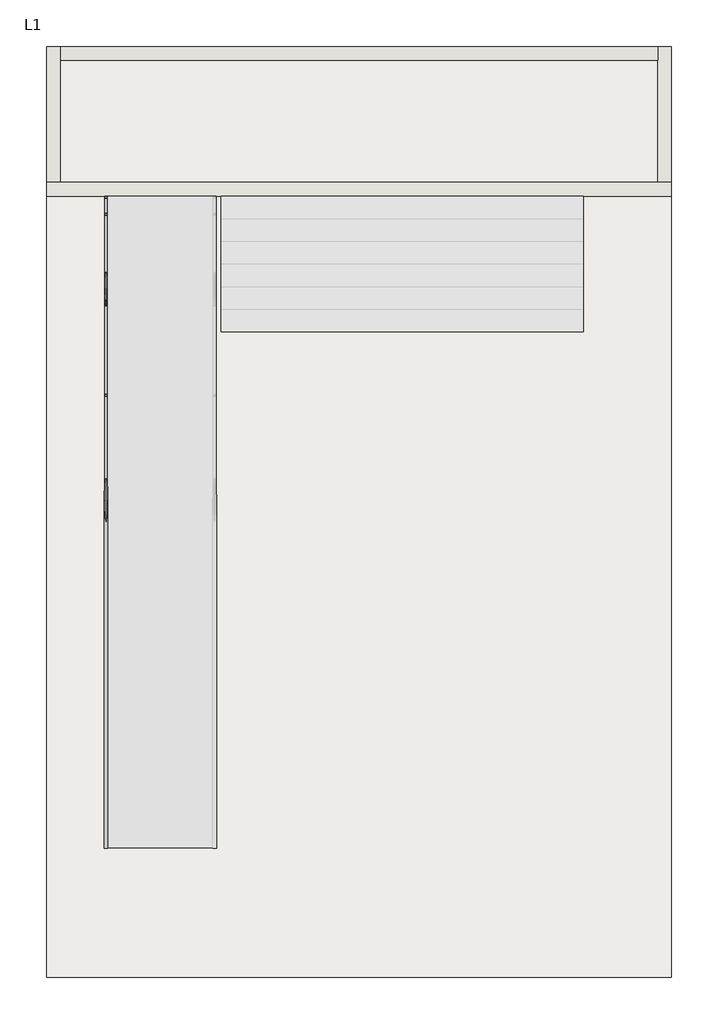
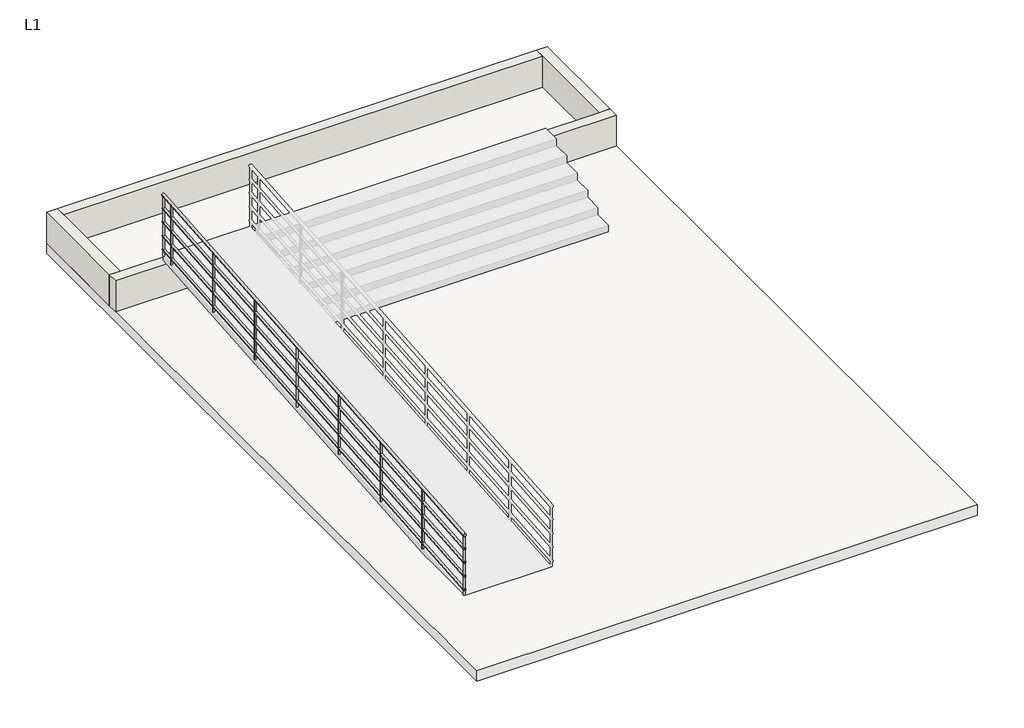
# One storey, part 1 of 2: 4 walls, 1 railing, 1 slab.
"""IFC4 building model written with IfcOpenShell, lengths in millimetres."""

from ifc_helpers import new_model, si_unit, frame, origin, origin_with_axes, place, context, project, spatial, polyline, ellipse_curve, outline, extrude, faceted_brep, element, save
from ifc_brep_helpers import plane_surface, cylinder_surface, advanced_brep

model = new_model("IFC4")

# Units and contexts
model_context = context("Model", 3, world=origin())
ifc_project = project(units=[si_unit("LENGTHUNIT", "METRE", prefix="MILLI")], contexts=[model_context])

# Site, building, storey
site = spatial("IfcSite", under=ifc_project)
building = spatial("IfcBuilding", under=site)
storey = spatial("IfcBuildingStorey", under=building, Name="L1", Elevation=0.0)

# Railing
placement = place(None, origin())
element("IfcRailing", 1, ObjectType="900mm Pipe", at=placement, inside=storey, context=model_context, shape_type="AdvancedBrep", body=[
    advanced_brep(
    [(-579.8488078, -8058.4292912, 879.9306757), (-619.8488078, -8058.4292912, 879.9306757), (-579.8488078, -858.4292912, 1479.9306757), (-619.8488078, -858.4292912, 1479.9306757)],
    [
        (0, 1, ellipse_curve(frame((-599.8488078, -8058.4292912, 879.9306757), z_axis=(0.0, -1.0, 0.0), x_axis=(0.0, 0.0, -1.0)), 20.0693243, 20.0)),
        (1, 0, ellipse_curve(frame((-599.8488078, -8058.4292912, 879.9306757), z_axis=(0.0, -1.0, 0.0), x_axis=(0.0, 0.0, -1.0)), 20.0693243, 20.0)),
        (2, 3, ellipse_curve(frame((-599.8488078, -858.4292912, 1479.9306757), z_axis=(0.0, 1.0, 0.0), x_axis=(0.0, 0.0, -1.0)), 20.0693243, 20.0)),
        (3, 2, ellipse_curve(frame((-599.8488078, -858.4292912, 1479.9306757), z_axis=(0.0, 1.0, 0.0), x_axis=(0.0, 0.0, -1.0)), 20.0693243, 20.0)),
        (0, 2),
        (3, 1),
    ],
    [
        plane_surface(frame((-599.8488078, -8058.4292912, 900.0), z_axis=(0.0, -1.0, 0.0), x_axis=(0.0, 0.0, 1.0))),
        plane_surface(frame((-599.8488078, -858.4292912, 1500.0), z_axis=(0.0, 1.0, 0.0), x_axis=(0.0, 0.0, 1.0))),
        cylinder_surface(frame((-599.8488078, -8056.7683816, 880.0690848), z_axis=(0.0, -0.9965457582448797, -0.08304547985373999), x_axis=(-1.0, 0.0, 0.0)), 20.0),
    ],
    [
        (0, [[1, 2]]),
        (1, [[3, 4]]),
        (2, [[-1, 5, -4, 6]]),
        (2, [[-2, -6, -3, -5]]),
    ],
),
    advanced_brep(
    [(-614.8488078, -8058.4292912, 684.9480068), (-584.8488078, -8058.4292912, 684.9480068), (-614.8488078, -858.4292912, 1284.9480068), (-584.8488078, -858.4292912, 1284.9480068)],
    [
        (0, 1, ellipse_curve(frame((-599.8488078, -8058.4292912, 684.9480068), z_axis=(0.0, -1.0, 0.0), x_axis=(0.0, 0.0, -0.9999999999999999)), 15.0519932, 15.0)),
        (1, 0, ellipse_curve(frame((-599.8488078, -8058.4292912, 684.9480068), z_axis=(0.0, -1.0, 0.0), x_axis=(0.0, 0.0, -0.9999999999999999)), 15.0519932, 15.0)),
        (2, 3, ellipse_curve(frame((-599.8488078, -858.4292912, 1284.9480068), z_axis=(0.0, 1.0, 0.0), x_axis=(0.0, 0.0, -0.9999999999999999)), 15.0519932, 15.0)),
        (3, 2, ellipse_curve(frame((-599.8488078, -858.4292912, 1284.9480068), z_axis=(0.0, 1.0, 0.0), x_axis=(0.0, 0.0, -0.9999999999999999)), 15.0519932, 15.0)),
        (0, 2),
        (3, 1),
    ],
    [
        plane_surface(frame((-599.8488078, -8058.4292912, 700.0), z_axis=(0.0, -1.0, 0.0), x_axis=(0.0, 0.0, 1.0))),
        plane_surface(frame((-599.8488078, -858.4292912, 1300.0), z_axis=(0.0, 1.0, 0.0), x_axis=(0.0, 0.0, 1.0))),
        cylinder_surface(frame((-599.8488078, -8057.183609, 685.0518136), z_axis=(0.0, -0.9965457582448797, -0.08304547985373997), x_axis=(1.0, 0.0, 0.0)), 15.0),
    ],
    [
        (0, [[1, 2]]),
        (1, [[3, 4]]),
        (2, [[-1, 5, -4, 6]]),
        (2, [[-2, -6, -3, -5]]),
    ],
),
    advanced_brep(
    [(-614.8488078, -8058.4292912, 484.9480068), (-584.8488078, -8058.4292912, 484.9480068), (-614.8488078, -858.4292912, 1084.9480068), (-584.8488078, -858.4292912, 1084.9480068)],
    [
        (0, 1, ellipse_curve(frame((-599.8488078, -8058.4292912, 484.9480068), z_axis=(0.0, -1.0, 0.0), x_axis=(0.0, 0.0, -0.9999999999999999)), 15.0519932, 15.0)),
        (1, 0, ellipse_curve(frame((-599.8488078, -8058.4292912, 484.9480068), z_axis=(0.0, -1.0, 0.0), x_axis=(0.0, 0.0, -0.9999999999999999)), 15.0519932, 15.0)),
        (2, 3, ellipse_curve(frame((-599.8488078, -858.4292912, 1084.9480068), z_axis=(0.0, 1.0, 0.0), x_axis=(0.0, 0.0, -0.9999999999999999)), 15.0519932, 15.0)),
        (3, 2, ellipse_curve(frame((-599.8488078, -858.4292912, 1084.9480068), z_axis=(0.0, 1.0, 0.0), x_axis=(0.0, 0.0, -0.9999999999999999)), 15.0519932, 15.0)),
        (0, 2),
        (3, 1),
    ],
    [
        plane_surface(frame((-599.8488078, -8058.4292912, 500.0), z_axis=(0.0, -1.0, 0.0), x_axis=(0.0, 0.0, 1.0))),
        plane_surface(frame((-599.8488078, -858.4292912, 1100.0), z_axis=(0.0, 1.0, 0.0), x_axis=(0.0, 0.0, 1.0))),
        cylinder_surface(frame((-599.8488078, -8057.183609, 485.0518136), z_axis=(0.0, -0.9965457582448797, -0.08304547985373997), x_axis=(1.0, 0.0, 0.0)), 15.0),
    ],
    [
        (0, [[1, 2]]),
        (1, [[3, 4]]),
        (2, [[-1, 5, -4, 6]]),
        (2, [[-2, -6, -3, -5]]),
    ],
),
    advanced_brep(
    [(-614.8488078, -8058.4292912, 284.9480068), (-584.8488078, -8058.4292912, 284.9480068), (-614.8488078, -858.4292912, 884.9480068), (-584.8488078, -858.4292912, 884.9480068)],
    [
        (0, 1, ellipse_curve(frame((-599.8488078, -8058.4292912, 284.9480068), z_axis=(0.0, -1.0, 0.0), x_axis=(0.0, 0.0, -0.9999999999999999)), 15.0519932, 15.0)),
        (1, 0, ellipse_curve(frame((-599.8488078, -8058.4292912, 284.9480068), z_axis=(0.0, -1.0, 0.0), x_axis=(0.0, 0.0, -0.9999999999999999)), 15.0519932, 15.0)),
        (2, 3, ellipse_curve(frame((-599.8488078, -858.4292912, 884.9480068), z_axis=(0.0, 1.0, 0.0), x_axis=(0.0, 0.0, -0.9999999999999999)), 15.0519932, 15.0)),
        (3, 2, ellipse_curve(frame((-599.8488078, -858.4292912, 884.9480068), z_axis=(0.0, 1.0, 0.0), x_axis=(0.0, 0.0, -0.9999999999999999)), 15.0519932, 15.0)),
        (0, 2),
        (3, 1),
    ],
    [
        plane_surface(frame((-599.8488078, -8058.4292912, 300.0), z_axis=(0.0, -1.0, 0.0), x_axis=(0.0, 0.0, 1.0))),
        plane_surface(frame((-599.8488078, -858.4292912, 900.0), z_axis=(0.0, 1.0, 0.0), x_axis=(0.0, 0.0, 1.0))),
        cylinder_surface(frame((-599.8488078, -8057.183609, 285.0518136), z_axis=(0.0, -0.9965457582448797, -0.08304547985373997), x_axis=(1.0, 0.0, 0.0)), 15.0),
    ],
    [
        (0, [[1, 2]]),
        (1, [[3, 4]]),
        (2, [[-1, 5, -4, 6]]),
        (2, [[-2, -6, -3, -5]]),
    ],
),
    advanced_brep(
    [(-614.8488078, -8058.4292912, 84.9480068), (-584.8488078, -8058.4292912, 84.9480068), (-614.8488078, -858.4292912, 684.9480068), (-584.8488078, -858.4292912, 684.9480068)],
    [
        (0, 1, ellipse_curve(frame((-599.8488078, -8058.4292912, 84.9480068), z_axis=(0.0, -1.0, 0.0), x_axis=(0.0, 0.0, -0.9999999999999999)), 15.0519932, 15.0)),
        (1, 0, ellipse_curve(frame((-599.8488078, -8058.4292912, 84.9480068), z_axis=(0.0, -1.0, 0.0), x_axis=(0.0, 0.0, -0.9999999999999999)), 15.0519932, 15.0)),
        (2, 3, ellipse_curve(frame((-599.8488078, -858.4292912, 684.9480068), z_axis=(0.0, 1.0, 0.0), x_axis=(0.0, 0.0, -0.9999999999999999)), 15.0519932, 15.0)),
        (3, 2, ellipse_curve(frame((-599.8488078, -858.4292912, 684.9480068), z_axis=(0.0, 1.0, 0.0), x_axis=(0.0, 0.0, -0.9999999999999999)), 15.0519932, 15.0)),
        (0, 2),
        (3, 1),
    ],
    [
        plane_surface(frame((-599.8488078, -8058.4292912, 100.0), z_axis=(0.0, -1.0, 0.0), x_axis=(0.0, 0.0, 1.0))),
        plane_surface(frame((-599.8488078, -858.4292912, 700.0), z_axis=(0.0, 1.0, 0.0), x_axis=(0.0, 0.0, 1.0))),
        cylinder_surface(frame((-599.8488078, -8057.183609, 85.0518136), z_axis=(0.0, -0.9965457582448797, -0.08304547985373997), x_axis=(1.0, 0.0, 0.0)), 15.0),
    ],
    [
        (0, [[1, 2]]),
        (1, [[3, 4]]),
        (2, [[-1, 5, -4, 6]]),
        (2, [[-2, -6, -3, -5]]),
    ],
),
    advanced_brep(
    [(-587.3488078, -1058.4292912, 1443.1946847), (-587.3488078, -1058.4292912, 583.3333333), (-612.3488078, -1058.4292912, 583.3333333), (-612.3488078, -1058.4292912, 1443.1946847)],
    [
        (0, 1),
        (1, 2, ellipse_curve(frame((-599.8488078, -1058.4292912, 583.3333333), z_axis=(0.0, -0.08304547985373995, 0.9965457582448797), x_axis=(0.0, 0.9965457582448798, 0.08304547985373882)), 12.5433277, 12.5)),
        (2, 3),
        (3, 0, ellipse_curve(frame((-599.8488078, -1058.4292912, 1443.1946847), z_axis=(0.0, 0.08304547985373997, -0.9965457582448797), x_axis=(0.0, 0.9965457582448797, 0.0830454798537388)), 12.5433277, 12.5)),
        (0, 3, ellipse_curve(frame((-599.8488078, -1058.4292912, 1443.1946847), z_axis=(0.0, 0.08304547985373997, -0.9965457582448797), x_axis=(0.0, 0.9965457582448797, 0.0830454798537388)), 12.5433277, 12.5)),
        (2, 1, ellipse_curve(frame((-599.8488078, -1058.4292912, 583.3333333), z_axis=(0.0, -0.08304547985373995, 0.9965457582448797), x_axis=(0.0, 0.9965457582448798, 0.08304547985373882)), 12.5433277, 12.5)),
    ],
    [
        cylinder_surface(frame((-599.8488078, -1058.4292912, 483.3333333), z_axis=(0.0, 0.0, 1.0), x_axis=(-1.0, 0.0, 0.0)), 12.5),
        plane_surface(frame((-624.8488078, -1033.4292912, 1445.2780181), z_axis=(0.0, -0.08304547985373997, 0.9965457582448797), x_axis=(1.0, 0.0, 0.0))),
        plane_surface(frame((-624.8488078, -1083.4292912, 581.25), z_axis=(0.0, 0.08304547985373995, -0.9965457582448797), x_axis=(1.0, 0.0, 0.0))),
    ],
    [
        (0, [[1, 2, 3, 4]]),
        (0, [[-1, 5, -3, 6]]),
        (1, [[-4, -5]]),
        (2, [[-2, -6]]),
    ],
),
    advanced_brep(
    [(-587.3488078, -2058.4292912, 1359.8613514), (-587.3488078, -2058.4292912, 500.0), (-612.3488078, -2058.4292912, 500.0), (-612.3488078, -2058.4292912, 1359.8613514)],
    [
        (0, 1),
        (1, 2, ellipse_curve(frame((-599.8488078, -2058.4292912, 500.0), z_axis=(0.0, -0.08304547985373995, 0.9965457582448797), x_axis=(0.0, 0.9965457582448798, 0.08304547985373882)), 12.5433277, 12.5)),
        (2, 3),
        (3, 0, ellipse_curve(frame((-599.8488078, -2058.4292912, 1359.8613514), z_axis=(0.0, 0.08304547985373997, -0.9965457582448797), x_axis=(0.0, 0.9965457582448797, 0.0830454798537388)), 12.5433277, 12.5)),
        (0, 3, ellipse_curve(frame((-599.8488078, -2058.4292912, 1359.8613514), z_axis=(0.0, 0.08304547985373997, -0.9965457582448797), x_axis=(0.0, 0.9965457582448797, 0.0830454798537388)), 12.5433277, 12.5)),
        (2, 1, ellipse_curve(frame((-599.8488078, -2058.4292912, 500.0), z_axis=(0.0, -0.08304547985373995, 0.9965457582448797), x_axis=(0.0, 0.9965457582448798, 0.08304547985373882)), 12.5433277, 12.5)),
    ],
    [
        cylinder_surface(frame((-599.8488078, -2058.4292912, 400.0), z_axis=(0.0, 0.0, 1.0), x_axis=(-1.0, 0.0, 0.0)), 12.5),
        plane_surface(frame((-624.8488078, -2033.4292912, 1361.9446847), z_axis=(0.0, -0.08304547985373997, 0.9965457582448797), x_axis=(1.0, 0.0, 0.0))),
        plane_surface(frame((-624.8488078, -2083.4292912, 497.9166667), z_axis=(0.0, 0.08304547985373995, -0.9965457582448797), x_axis=(1.0, 0.0, 0.0))),
    ],
    [
        (0, [[1, 2, 3, 4]]),
        (0, [[-1, 5, -3, 6]]),
        (1, [[-4, -5]]),
        (2, [[-2, -6]]),
    ],
),
    advanced_brep(
    [(-587.3488078, -3058.4292912, 1276.5280181), (-587.3488078, -3058.4292912, 416.6666667), (-612.3488078, -3058.4292912, 416.6666667), (-612.3488078, -3058.4292912, 1276.5280181)],
    [
        (0, 1),
        (1, 2, ellipse_curve(frame((-599.8488078, -3058.4292912, 416.6666667), z_axis=(0.0, -0.08304547985373995, 0.9965457582448797), x_axis=(0.0, 0.9965457582448798, 0.08304547985373882)), 12.5433277, 12.5)),
        (2, 3),
        (3, 0, ellipse_curve(frame((-599.8488078, -3058.4292912, 1276.5280181), z_axis=(0.0, 0.08304547985373997, -0.9965457582448797), x_axis=(0.0, 0.9965457582448797, 0.0830454798537388)), 12.5433277, 12.5)),
        (0, 3, ellipse_curve(frame((-599.8488078, -3058.4292912, 1276.5280181), z_axis=(0.0, 0.08304547985373997, -0.9965457582448797), x_axis=(0.0, 0.9965457582448797, 0.0830454798537388)), 12.5433277, 12.5)),
        (2, 1, ellipse_curve(frame((-599.8488078, -3058.4292912, 416.6666667), z_axis=(0.0, -0.08304547985373995, 0.9965457582448797), x_axis=(0.0, 0.9965457582448798, 0.08304547985373882)), 12.5433277, 12.5)),
    ],
    [
        cylinder_surface(frame((-599.8488078, -3058.4292912, 316.6666667), z_axis=(0.0, 0.0, 1.0), x_axis=(-1.0, 0.0, 0.0)), 12.5),
        plane_surface(frame((-624.8488078, -3033.4292912, 1278.6113514), z_axis=(0.0, -0.08304547985373997, 0.9965457582448797), x_axis=(1.0, 0.0, 0.0))),
        plane_surface(frame((-624.8488078, -3083.4292912, 414.5833333), z_axis=(0.0, 0.08304547985373995, -0.9965457582448797), x_axis=(1.0, 0.0, 0.0))),
    ],
    [
        (0, [[1, 2, 3, 4]]),
        (0, [[-1, 5, -3, 6]]),
        (1, [[-4, -5]]),
        (2, [[-2, -6]]),
    ],
),
    advanced_brep(
    [(-587.3488078, -4058.4292912, 1193.1946847), (-587.3488078, -4058.4292912, 333.3333333), (-612.3488078, -4058.4292912, 333.3333333), (-612.3488078, -4058.4292912, 1193.1946847)],
    [
        (0, 1),
        (1, 2, ellipse_curve(frame((-599.8488078, -4058.4292912, 333.3333333), z_axis=(0.0, -0.08304547985373995, 0.9965457582448797), x_axis=(0.0, 0.9965457582448798, 0.08304547985373882)), 12.5433277, 12.5)),
        (2, 3),
        (3, 0, ellipse_curve(frame((-599.8488078, -4058.4292912, 1193.1946847), z_axis=(0.0, 0.08304547985373997, -0.9965457582448797), x_axis=(0.0, 0.9965457582448797, 0.0830454798537388)), 12.5433277, 12.5)),
        (0, 3, ellipse_curve(frame((-599.8488078, -4058.4292912, 1193.1946847), z_axis=(0.0, 0.08304547985373997, -0.9965457582448797), x_axis=(0.0, 0.9965457582448797, 0.0830454798537388)), 12.5433277, 12.5)),
        (2, 1, ellipse_curve(frame((-599.8488078, -4058.4292912, 333.3333333), z_axis=(0.0, -0.08304547985373995, 0.9965457582448797), x_axis=(0.0, 0.9965457582448798, 0.08304547985373882)), 12.5433277, 12.5)),
    ],
    [
        cylinder_surface(frame((-599.8488078, -4058.4292912, 233.3333333), z_axis=(0.0, 0.0, 1.0), x_axis=(-1.0, 0.0, 0.0)), 12.5),
        plane_surface(frame((-624.8488078, -4033.4292912, 1195.2780181), z_axis=(0.0, -0.08304547985373997, 0.9965457582448797), x_axis=(1.0, 0.0, 0.0))),
        plane_surface(frame((-624.8488078, -4083.4292912, 331.25), z_axis=(0.0, 0.08304547985373995, -0.9965457582448797), x_axis=(1.0, 0.0, 0.0))),
    ],
    [
        (0, [[1, 2, 3, 4]]),
        (0, [[-1, 5, -3, 6]]),
        (1, [[-4, -5]]),
        (2, [[-2, -6]]),
    ],
),
    advanced_brep(
    [(-587.3488078, -5058.4292912, 1109.8613514), (-587.3488078, -5058.4292912, 250.0), (-612.3488078, -5058.4292912, 250.0), (-612.3488078, -5058.4292912, 1109.8613514)],
    [
        (0, 1),
        (1, 2, ellipse_curve(frame((-599.8488078, -5058.4292912, 250.0), z_axis=(0.0, -0.08304547985373995, 0.9965457582448797), x_axis=(0.0, 0.9965457582448798, 0.08304547985373882)), 12.5433277, 12.5)),
        (2, 3),
        (3, 0, ellipse_curve(frame((-599.8488078, -5058.4292912, 1109.8613514), z_axis=(0.0, 0.08304547985373997, -0.9965457582448797), x_axis=(0.0, 0.9965457582448797, 0.0830454798537388)), 12.5433277, 12.5)),
        (0, 3, ellipse_curve(frame((-599.8488078, -5058.4292912, 1109.8613514), z_axis=(0.0, 0.08304547985373997, -0.9965457582448797), x_axis=(0.0, 0.9965457582448797, 0.0830454798537388)), 12.5433277, 12.5)),
        (2, 1, ellipse_curve(frame((-599.8488078, -5058.4292912, 250.0), z_axis=(0.0, -0.08304547985373995, 0.9965457582448797), x_axis=(0.0, 0.9965457582448798, 0.08304547985373882)), 12.5433277, 12.5)),
    ],
    [
        cylinder_surface(frame((-599.8488078, -5058.4292912, 150.0), z_axis=(0.0, 0.0, 1.0), x_axis=(-1.0, 0.0, 0.0)), 12.5),
        plane_surface(frame((-624.8488078, -5033.4292912, 1111.9446847), z_axis=(0.0, -0.08304547985373997, 0.9965457582448797), x_axis=(1.0, 0.0, 0.0))),
        plane_surface(frame((-624.8488078, -5083.4292912, 247.9166667), z_axis=(0.0, 0.08304547985373995, -0.9965457582448797), x_axis=(1.0, 0.0, 0.0))),
    ],
    [
        (0, [[1, 2, 3, 4]]),
        (0, [[-1, 5, -3, 6]]),
        (1, [[-4, -5]]),
        (2, [[-2, -6]]),
    ],
),
    advanced_brep(
    [(-587.3488078, -6058.4292912, 1026.5280181), (-587.3488078, -6058.4292912, 166.6666667), (-612.3488078, -6058.4292912, 166.6666667), (-612.3488078, -6058.4292912, 1026.5280181)],
    [
        (0, 1),
        (1, 2, ellipse_curve(frame((-599.8488078, -6058.4292912, 166.6666667), z_axis=(0.0, -0.08304547985373995, 0.9965457582448797), x_axis=(0.0, 0.9965457582448798, 0.08304547985373882)), 12.5433277, 12.5)),
        (2, 3),
        (3, 0, ellipse_curve(frame((-599.8488078, -6058.4292912, 1026.5280181), z_axis=(0.0, 0.08304547985373997, -0.9965457582448797), x_axis=(0.0, 0.9965457582448797, 0.0830454798537388)), 12.5433277, 12.5)),
        (0, 3, ellipse_curve(frame((-599.8488078, -6058.4292912, 1026.5280181), z_axis=(0.0, 0.08304547985373997, -0.9965457582448797), x_axis=(0.0, 0.9965457582448797, 0.0830454798537388)), 12.5433277, 12.5)),
        (2, 1, ellipse_curve(frame((-599.8488078, -6058.4292912, 166.6666667), z_axis=(0.0, -0.08304547985373995, 0.9965457582448797), x_axis=(0.0, 0.9965457582448798, 0.08304547985373882)), 12.5433277, 12.5)),
    ],
    [
        cylinder_surface(frame((-599.8488078, -6058.4292912, 66.6666667), z_axis=(0.0, 0.0, 1.0), x_axis=(-1.0, 0.0, 0.0)), 12.5),
        plane_surface(frame((-624.8488078, -6033.4292912, 1028.6113514), z_axis=(0.0, -0.08304547985373997, 0.9965457582448797), x_axis=(1.0, 0.0, 0.0))),
        plane_surface(frame((-624.8488078, -6083.4292912, 164.5833333), z_axis=(0.0, 0.08304547985373995, -0.9965457582448797), x_axis=(1.0, 0.0, 0.0))),
    ],
    [
        (0, [[1, 2, 3, 4]]),
        (0, [[-1, 5, -3, 6]]),
        (1, [[-4, -5]]),
        (2, [[-2, -6]]),
    ],
),
    advanced_brep(
    [(-587.3488078, -7058.4292912, 943.1946847), (-587.3488078, -7058.4292912, 83.3333333), (-612.3488078, -7058.4292912, 83.3333333), (-612.3488078, -7058.4292912, 943.1946847)],
    [
        (0, 1),
        (1, 2, ellipse_curve(frame((-599.8488078, -7058.4292912, 83.3333333), z_axis=(0.0, -0.08304547985373995, 0.9965457582448797), x_axis=(0.0, 0.9965457582448798, 0.08304547985373882)), 12.5433277, 12.5)),
        (2, 3),
        (3, 0, ellipse_curve(frame((-599.8488078, -7058.4292912, 943.1946847), z_axis=(0.0, 0.08304547985373997, -0.9965457582448797), x_axis=(0.0, 0.9965457582448797, 0.0830454798537388)), 12.5433277, 12.5)),
        (0, 3, ellipse_curve(frame((-599.8488078, -7058.4292912, 943.1946847), z_axis=(0.0, 0.08304547985373997, -0.9965457582448797), x_axis=(0.0, 0.9965457582448797, 0.0830454798537388)), 12.5433277, 12.5)),
        (2, 1, ellipse_curve(frame((-599.8488078, -7058.4292912, 83.3333333), z_axis=(0.0, -0.08304547985373995, 0.9965457582448797), x_axis=(0.0, 0.9965457582448798, 0.08304547985373882)), 12.5433277, 12.5)),
    ],
    [
        cylinder_surface(frame((-599.8488078, -7058.4292912, -16.6666667), z_axis=(0.0, 0.0, 1.0), x_axis=(-1.0, 0.0, 0.0)), 12.5),
        plane_surface(frame((-624.8488078, -7033.4292912, 945.2780181), z_axis=(0.0, -0.08304547985373997, 0.9965457582448797), x_axis=(1.0, 0.0, 0.0))),
        plane_surface(frame((-624.8488078, -7083.4292912, 81.25), z_axis=(0.0, 0.08304547985373995, -0.9965457582448797), x_axis=(1.0, 0.0, 0.0))),
    ],
    [
        (0, [[1, 2, 3, 4]]),
        (0, [[-1, 5, -3, 6]]),
        (1, [[-4, -5]]),
        (2, [[-2, -6]]),
    ],
),
    advanced_brep(
    [(-587.3488078, -870.9292912, 1458.8196847), (-587.3488078, -870.9292912, 598.9583333), (-612.3488078, -870.9292912, 598.9583333), (-612.3488078, -870.9292912, 1458.8196847)],
    [
        (0, 1),
        (1, 2, ellipse_curve(frame((-599.8488078, -870.9292912, 598.9583333), z_axis=(0.0, -0.08304547985373995, 0.9965457582448797), x_axis=(0.0, 0.9965457582448798, 0.08304547985373882)), 12.5433277, 12.5)),
        (2, 3),
        (3, 0, ellipse_curve(frame((-599.8488078, -870.9292912, 1458.8196847), z_axis=(0.0, 0.08304547985373997, -0.9965457582448797), x_axis=(0.0, 0.9965457582448797, 0.0830454798537388)), 12.5433277, 12.5)),
        (0, 3, ellipse_curve(frame((-599.8488078, -870.9292912, 1458.8196847), z_axis=(0.0, 0.08304547985373997, -0.9965457582448797), x_axis=(0.0, 0.9965457582448797, 0.0830454798537388)), 12.5433277, 12.5)),
        (2, 1, ellipse_curve(frame((-599.8488078, -870.9292912, 598.9583333), z_axis=(0.0, -0.08304547985373995, 0.9965457582448797), x_axis=(0.0, 0.9965457582448798, 0.08304547985373882)), 12.5433277, 12.5)),
    ],
    [
        cylinder_surface(frame((-599.8488078, -870.9292912, 498.9583333), z_axis=(0.0, 0.0, 1.0), x_axis=(-1.0, 0.0, 0.0)), 12.5),
        plane_surface(frame((-624.8488078, -845.9292912, 1460.9030181), z_axis=(0.0, -0.08304547985373997, 0.9965457582448797), x_axis=(1.0, 0.0, 0.0))),
        plane_surface(frame((-624.8488078, -895.9292912, 596.875), z_axis=(0.0, 0.08304547985373995, -0.9965457582448797), x_axis=(1.0, 0.0, 0.0))),
    ],
    [
        (0, [[1, 2, 3, 4]]),
        (0, [[-1, 5, -3, 6]]),
        (1, [[-4, -5]]),
        (2, [[-2, -6]]),
    ],
),
    advanced_brep(
    [(-587.3488078, -8045.9292912, 860.9030181), (-587.3488078, -8045.9292912, 1.0416667), (-612.3488078, -8045.9292912, 1.0416667), (-612.3488078, -8045.9292912, 860.9030181)],
    [
        (0, 1),
        (1, 2, ellipse_curve(frame((-599.8488078, -8045.9292912, 1.0416667), z_axis=(0.0, -0.08304547985373995, 0.9965457582448797), x_axis=(0.0, 0.9965457582448798, 0.08304547985373882)), 12.5433277, 12.5)),
        (2, 3),
        (3, 0, ellipse_curve(frame((-599.8488078, -8045.9292912, 860.9030181), z_axis=(0.0, 0.08304547985373997, -0.9965457582448797), x_axis=(0.0, 0.9965457582448797, 0.0830454798537388)), 12.5433277, 12.5)),
        (0, 3, ellipse_curve(frame((-599.8488078, -8045.9292912, 860.9030181), z_axis=(0.0, 0.08304547985373997, -0.9965457582448797), x_axis=(0.0, 0.9965457582448797, 0.0830454798537388)), 12.5433277, 12.5)),
        (2, 1, ellipse_curve(frame((-599.8488078, -8045.9292912, 1.0416667), z_axis=(0.0, -0.08304547985373995, 0.9965457582448797), x_axis=(0.0, 0.9965457582448798, 0.08304547985373882)), 12.5433277, 12.5)),
    ],
    [
        cylinder_surface(frame((-599.8488078, -8045.9292912, -98.9583333), z_axis=(0.0, 0.0, 1.0), x_axis=(-1.0, 0.0, 0.0)), 12.5),
        plane_surface(frame((-624.8488078, -8020.9292912, 862.9863514), z_axis=(0.0, -0.08304547985373997, 0.9965457582448797), x_axis=(1.0, 0.0, 0.0))),
        plane_surface(frame((-624.8488078, -8070.9292912, -1.0416667), z_axis=(0.0, 0.08304547985373995, -0.9965457582448797), x_axis=(1.0, 0.0, 0.0))),
    ],
    [
        (0, [[1, 2, 3, 4]]),
        (0, [[-1, 5, -3, 6]]),
        (1, [[-4, -5]]),
        (2, [[-2, -6]]),
    ],
),
])

# Slab
element("IfcSlab", 2, ObjectType="Concrete 150mm", at=placement, inside=storey, context=model_context, shape_type="SweptSolid", body=[
    extrude(outline(polyline([(5643.2318, -9483.4292912), (-1256.7682, -9483.4292912), (-1256.7682, 791.5707088), (5643.2318, 791.5707088), (5643.2318, -9483.4292912)])), frame((0.0, 0.0, -150.0), z_axis=(0.0, 0.0, 1.0), x_axis=(1.0, 0.0, 0.0)), (0.0, 0.0, 1.0), 150.0),
])

# Walls
element("IfcWall", 3, ObjectType="Generic - 150mm", at=placement, inside=storey, context=model_context, shape_type="Brep", body=[
    faceted_brep([(-1256.7682, -858.4292912, 0.0), (5643.2318, -858.4292912, 0.0), (5643.2318, -858.4292912, 450.0), (-1256.7682, -858.4292912, 450.0), (-1256.7682, -708.4292912, 0.0), (-1256.7682, -708.4292912, 450.0), (-1106.7682, -708.4292912, 450.0), (5493.2318, -708.4292912, 450.0), (5643.2318, -708.4292912, 450.0), (5643.2318, -708.4292912, 0.0), (5493.2318, -708.4292912, 0.0), (-1106.7682, -708.4292912, 0.0)], [[[0, 1, 2, 3]], [[4, 5, 6, 7, 8, 9, 10, 11]], [[1, 0, 4, 11, 10, 9]], [[3, 2, 8, 7, 6, 5]], [[0, 3, 5, 4]], [[2, 1, 9, 8]]]),
])
element("IfcWall", 4, ObjectType="Generic - 150mm", at=placement, inside=storey, context=model_context, shape_type="Brep", body=[
    faceted_brep([(-1106.7682, -708.4292912, 0.0), (-1106.7682, 641.5707088, 0.0), (-1106.7682, 791.5707088, 0.0), (-1106.7682, 791.5707088, 450.0), (-1106.7682, 641.5707088, 450.0), (-1106.7682, -708.4292912, 450.0), (-1256.7682, -708.4292912, 0.0), (-1256.7682, -708.4292912, 450.0), (-1256.7682, 791.5707088, 450.0), (-1256.7682, 791.5707088, 0.0)], [[[0, 1, 2, 3, 4, 5]], [[6, 7, 8, 9]], [[2, 1, 0, 6, 9]], [[5, 4, 3, 8, 7]], [[0, 5, 7, 6]], [[3, 2, 9, 8]]]),
])
element("IfcWall", 5, ObjectType="Generic - 150mm", at=placement, inside=storey, context=model_context, shape_type="Brep", body=[
    faceted_brep([(5643.2318, -708.4292912, 0.0), (5643.2318, 791.5707088, 0.0), (5643.2318, 791.5707088, 450.0), (5643.2318, -708.4292912, 450.0), (5493.2318, -708.4292912, 0.0), (5493.2318, -708.4292912, 450.0), (5493.2318, 641.5707088, 450.0), (5493.2318, 791.5707088, 450.0), (5493.2318, 791.5707088, 0.0), (5493.2318, 641.5707088, 0.0)], [[[0, 1, 2, 3]], [[4, 5, 6, 7, 8, 9]], [[1, 0, 4, 9, 8]], [[3, 2, 7, 6, 5]], [[0, 3, 5, 4]], [[2, 1, 8, 7]]]),
])
element("IfcWall", 6, ObjectType="Generic - 150mm", at=placement, inside=storey, context=model_context, shape_type="SweptSolid", body=[
    extrude(outline(polyline([(5493.2318, 641.5707088), (-1106.7682, 641.5707088), (-1106.7682, 791.5707088), (5493.2318, 791.5707088), (5493.2318, 641.5707088)])), origin_with_axes(), (0.0, 0.0, 1.0), 450.0),
])

save(model, "model.ifc")

# Revit data of these elements
# Project information
#   Organization Name = "Organization Name"
#   Organization Description = "Organization Description"
#   Building Name = "Building Name"
#   Project Issue Date = "Issue Date"
#   Project Status = "Project Status"
#   Client Name = "Client Name"
#   Project Address = "Enter address here\nAddress Line 2"
#   Project Name = "Project Name"
#   Project Number = "Project Number"
# Type "900mm Pipe"
#   built-in parameter 1008612 = 0.019685 (stored number, unit not read)
#   built-in parameter 1008611 = 0.0984252 (stored number, unit not read)
#   built-in parameter 1008609 = 3.28084 (stored number, unit not read)
#   built-in parameter 1008604 = 0.19685 (stored number, unit not read)
#   built-in parameter 1008603 = 0.164042 (stored number, unit not read)
#   Railing Height = 900 mm
#   built-in parameter 1008630 = 2
#   built-in parameter 1008610 = 1
#   built-in parameter 1008605 = 1
#   built-in parameter 1008618 = M_Baluster - Round : 25mm
# Type "Concrete 150mm"
#   Description = "Concrete Floor, 100mm thick, Interior Function"
#   Type Mark = "SF01"
#   Function = 0
#   Layers, outside or top first: 150 mm "Concrete, Cast-in-Place gray" (function 1)
# Type "Generic - 150mm"
#   Description = "Generic Wall (Material By Category), 150mm thick"
#   Type Mark = "G04"
#   Layers, outside or top first: 150 mm no material (function 1)
# Element 1 (IfcRailing, "900mm Pipe")
#   Phase Created = New Construction
# Element 2 (IfcSlab, "Concrete 150mm")
#   Height Offset From Level = 0 mm
#   Phase Created = New Construction
#   Materials on its faces: "Concrete, Cast-in-Place gray"
# Element 3 (IfcWall, "Generic - 150mm")
#   Top Offset = 0 mm
#   Base Offset = 0 mm
#   wall height = 600 mm
#   Phase Created = New Construction
#   Base Constraint = L1
#   Top Constraint = L2
#   Materials on its faces: "Default Wall"
# Elements 4, 5, 6 (IfcWall, "Generic - 150mm")
#   Top Offset = 0 mm
#   Base Offset = 0 mm
#   Unconnected Height = 450 mm
#   wall height = 450 mm
#   Phase Created = New Construction
#   Base Constraint = L1
#   Materials on its faces: "Default Wall"
# Materials
#   "Concrete, Cast-in-Place gray": class "Concrete", colour RGB 192 192 192, transparency 0, Description = "Cast-in-place concrete", Cost = 0
#   "Default Wall": class "Miscellaneous", colour RGB 192 192 192, transparency 0, Cost = 0
